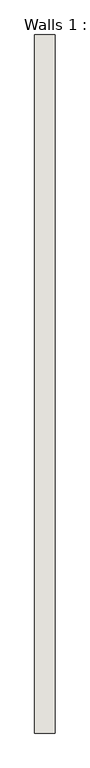
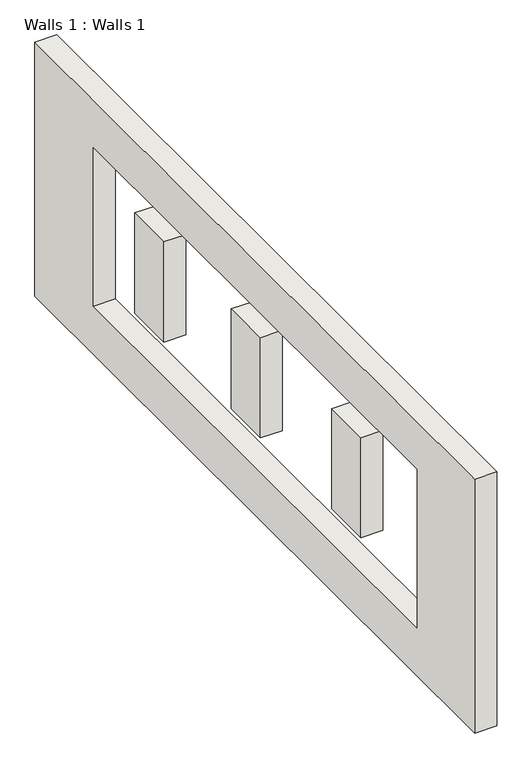
"""IFC4 building model written with IfcOpenShell, lengths in millimetres: wall geometry, Walls 1 : Walls 1."""

from ifc_helpers import new_model, si_unit, frame, origin, place, context, project, spatial, polyline, outline, extrude, source, transform, mapped, element, save


def walls_1_walls_1_17145d76(model_context):
    return source(origin(), model_context, "Body", "SweptSolid", [
        extrude(outline(polyline([(-4909.8784477, 1581.347646), (-4909.8784477, 364.147646), (-8364.2784477, 364.147646), (-8364.2784477, 1581.347646), (-4909.8784477, 1581.347646)]), holes=[polyline([(-5367.0784477, 1352.747646), (-7907.0784477, 1352.747646), (-7907.0784477, 592.747646), (-5367.0784477, 592.747646), (-5367.0784477, 1352.747646)])]), frame((27432.0, 0.0, 0.0), z_axis=(1.0, 0.0, 0.0), x_axis=(0.0, 1.0, 0.0)), (0.0, 0.0, 1.0), 100.0),
        extrude(outline(polyline([(27532.0, -7240.8779856), (27532.0, -7469.4779856), (27432.0, -7469.4779856), (27432.0, -7240.8779856), (27532.0, -7240.8779856)])), frame((0.0, 0.0, 758.3974408), z_axis=(0.0, 0.0, 1.0), x_axis=(1.0, 0.0, 0.0)), (0.0, 0.0, 1.0), 480.0),
        extrude(outline(polyline([(27532.0, -6452.0575733), (27532.0, -6680.6575733), (27432.0, -6680.6575733), (27432.0, -6452.0575733), (27532.0, -6452.0575733)])), frame((0.0, 0.0, 758.3974408), z_axis=(0.0, 0.0, 1.0), x_axis=(1.0, 0.0, 0.0)), (0.0, 0.0, 1.0), 480.0),
        extrude(outline(polyline([(27532.0, -5694.4158334), (27532.0, -5923.0158334), (27432.0, -5923.0158334), (27432.0, -5694.4158334), (27532.0, -5694.4158334)])), frame((0.0, 0.0, 758.3974408), z_axis=(0.0, 0.0, 1.0), x_axis=(1.0, 0.0, 0.0)), (0.0, 0.0, 1.0), 480.0),
    ])


if __name__ == "__main__":
    model = new_model("IFC4")
    model_context = context("Model", 3, world=origin())
    ifc_project = project(units=[si_unit("LENGTHUNIT", "METRE", prefix="MILLI")], contexts=[model_context])
    site = spatial("IfcSite", under=ifc_project)
    building = spatial("IfcBuilding", under=site)
    placement = place(None, origin())
    walls_1_walls_1_shape = walls_1_walls_1_17145d76(model_context)
    element("IfcWall", 1, ObjectType="Walls 1 : Walls 1", at=placement, inside=building, context=model_context, shape_type="MappedRepresentation", body=[
        mapped(walls_1_walls_1_shape, transform((0.0, 0.0, 0.0), x_axis=(1.0, 0.0, 0.0), y_axis=(0.0, 1.0, 0.0), z_axis=(0.0, 0.0, 1.0))),
    ])
    save(model, "model.ifc")

# Revit data of these elements
# Type "Walls 1 : Walls 1"
#   MAT-1 = P-1
# Element 1 (IfcWall, "Walls 1 : Walls 1")
#   Materials on its faces: "P-1"
# Materials
#   "P-1": class "Generic", colour RGB 120 120 120, transparency 0, Cost = 0
